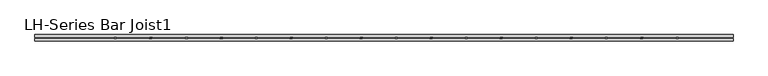
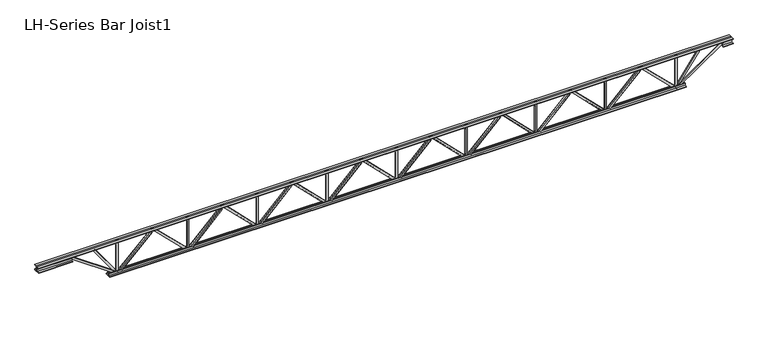
"""IFC4 building model written with IfcOpenShell, lengths in millimetres: beam geometry, LH-Series Bar Joist1 : 32LH-SP1."""

from ifc_helpers import new_model, si_unit, frame, origin, place, context, project, spatial, polyline, outline, extrude, faceted_brep, source, transform, mapped, element, save


def lh_series_bar_joist1_80182e71(model_context):
    return source(origin(), model_context, "Body", "SolidModel", [
        extrude(outline(polyline([(406.4, 3276.6), (406.4, 3225.8), (323.85, 3225.8), (312.7375, 3236.9125), (-312.7375, 3236.9125), (-323.85, 3225.8), (-406.4, 3225.8), (-406.4, 3276.6), (406.4, 3276.6)])), frame((0.0, -12.7, 0.0), z_axis=(0.0, 1.0, 0.0), x_axis=(0.0, 0.0, 1.0)), (0.0, 0.0, 1.0), 25.4),
        faceted_brep([(3251.2, 0.0, -355.6), (3251.2, 0.0, -406.4), (3251.2, 12.7, -406.4), (3251.2, 12.7, -355.6), (3236.3210245, 0.0, -355.6), (2474.3210245, 0.0, 406.4), (2413.0, 0.0, 406.4), (2413.0, 0.0, 355.6), (2453.2789755, 0.0, 355.6), (3215.2789755, 0.0, -406.4), (3215.2789755, 12.7, -406.4), (3151.7789755, 12.7, -342.9), (3160.7592316, 12.7, -333.9197439), (2474.9592316, 12.7, 351.8802561), (2465.9789755, 12.7, 342.9), (2453.2789755, 12.7, 355.6), (2413.0, 12.7, 355.6), (2413.0, 12.7, 406.4), (2474.3210245, 12.7, 406.4), (3236.3210245, 12.7, -355.6), (2465.9789755, 50.8, 342.9), (3151.7789755, 50.8, -342.9), (3160.7592316, 50.8, -333.9197439), (2474.9592316, 50.8, 351.8802561)], [[[0, 1, 2, 3]], [[1, 0, 4, 5, 6, 7, 8, 9]], [[2, 1, 9, 10]], [[3, 2, 10, 11, 12, 13, 14, 15, 16, 17, 18, 19]], [[0, 3, 19, 4]], [[9, 8, 15, 14, 20, 21, 11, 10]], [[5, 4, 19, 18]], [[7, 6, 17, 16]], [[8, 7, 16, 15]], [[6, 5, 18, 17]], [[11, 21, 22, 12]], [[13, 23, 20, 14]], [[22, 21, 20, 23]], [[12, 22, 23, 13]]]),
        faceted_brep([(1625.6, -12.7, -355.6), (1625.6, 0.0, -355.6), (1625.6, 0.0, -406.4), (1625.6, -12.7, -406.4), (1640.4789755, -12.7, -355.6), (1640.4789755, 0.0, -355.6), (2402.4789755, 0.0, 406.4), (2463.8, 0.0, 406.4), (2463.8, 0.0, 355.6), (2423.5210245, 0.0, 355.6), (1661.5210245, 0.0, -406.4), (1661.5210245, -12.7, -406.4), (1725.0210245, -12.7, -342.9), (1716.0407684, -12.7, -333.9197439), (2401.8407684, -12.7, 351.8802561), (2410.8210245, -12.7, 342.9), (2423.5210245, -12.7, 355.6), (2463.8, -12.7, 355.6), (2463.8, -12.7, 406.4), (2402.4789755, -12.7, 406.4), (2410.8210245, -50.8, 342.9), (1725.0210245, -50.8, -342.9), (1716.0407684, -50.8, -333.9197439), (2401.8407684, -50.8, 351.8802561)], [[[0, 1, 2, 3]], [[1, 0, 4, 5]], [[2, 1, 5, 6, 7, 8, 9, 10]], [[3, 2, 10, 11]], [[0, 3, 11, 12, 13, 14, 15, 16, 17, 18, 19, 4]], [[5, 4, 19, 6]], [[10, 9, 16, 15, 20, 21, 12, 11]], [[8, 7, 18, 17]], [[7, 6, 19, 18]], [[9, 8, 17, 16]], [[21, 22, 13, 12]], [[20, 15, 14, 23]], [[22, 21, 20, 23]], [[13, 22, 23, 14]]]),
        extrude(outline(polyline([(406.4, 1651.0), (406.4, 1600.2), (323.85, 1600.2), (312.7375, 1611.3125), (-312.7375, 1611.3125), (-323.85, 1600.2), (-406.4, 1600.2), (-406.4, 1651.0), (406.4, 1651.0)])), frame((0.0, -12.7, 0.0), z_axis=(0.0, 1.0, 0.0), x_axis=(0.0, 0.0, 1.0)), (0.0, 0.0, 1.0), 25.4),
        faceted_brep([(1625.6, 0.0, -355.6), (1625.6, 0.0, -406.4), (1625.6, 12.7, -406.4), (1625.6, 12.7, -355.6), (1610.7210245, 0.0, -355.6), (848.7210245, 0.0, 406.4), (787.4, 0.0, 406.4), (787.4, 0.0, 355.6), (827.6789755, 0.0, 355.6), (1589.6789755, 0.0, -406.4), (1589.6789755, 12.7, -406.4), (1526.1789755, 12.7, -342.9), (1535.1592316, 12.7, -333.9197439), (849.3592316, 12.7, 351.8802561), (840.3789755, 12.7, 342.9), (827.6789755, 12.7, 355.6), (787.4, 12.7, 355.6), (787.4, 12.7, 406.4), (848.7210245, 12.7, 406.4), (1610.7210245, 12.7, -355.6), (840.3789755, 50.8, 342.9), (1526.1789755, 50.8, -342.9), (1535.1592316, 50.8, -333.9197439), (849.3592316, 50.8, 351.8802561)], [[[0, 1, 2, 3]], [[1, 0, 4, 5, 6, 7, 8, 9]], [[2, 1, 9, 10]], [[3, 2, 10, 11, 12, 13, 14, 15, 16, 17, 18, 19]], [[0, 3, 19, 4]], [[9, 8, 15, 14, 20, 21, 11, 10]], [[5, 4, 19, 18]], [[7, 6, 17, 16]], [[8, 7, 16, 15]], [[6, 5, 18, 17]], [[11, 21, 22, 12]], [[13, 23, 20, 14]], [[22, 21, 20, 23]], [[12, 22, 23, 13]]]),
        faceted_brep([(0.0, -12.7, -355.6), (0.0, 0.0, -355.6), (0.0, 0.0, -406.4), (0.0, -12.7, -406.4), (14.8789755, -12.7, -355.6), (14.8789755, 0.0, -355.6), (776.8789755, 0.0, 406.4), (838.2, 0.0, 406.4), (838.2, 0.0, 355.6), (797.9210245, 0.0, 355.6), (35.9210245, 0.0, -406.4), (35.9210245, -12.7, -406.4), (99.4210245, -12.7, -342.9), (90.4407684, -12.7, -333.9197439), (776.2407684, -12.7, 351.8802561), (785.2210245, -12.7, 342.9), (797.9210245, -12.7, 355.6), (838.2, -12.7, 355.6), (838.2, -12.7, 406.4), (776.8789755, -12.7, 406.4), (785.2210245, -50.8, 342.9), (99.4210245, -50.8, -342.9), (90.4407684, -50.8, -333.9197439), (776.2407684, -50.8, 351.8802561)], [[[0, 1, 2, 3]], [[1, 0, 4, 5]], [[2, 1, 5, 6, 7, 8, 9, 10]], [[3, 2, 10, 11]], [[0, 3, 11, 12, 13, 14, 15, 16, 17, 18, 19, 4]], [[5, 4, 19, 6]], [[10, 9, 16, 15, 20, 21, 12, 11]], [[8, 7, 18, 17]], [[7, 6, 19, 18]], [[9, 8, 17, 16]], [[21, 22, 13, 12]], [[20, 15, 14, 23]], [[22, 21, 20, 23]], [[13, 22, 23, 14]]]),
        extrude(outline(polyline([(406.4, 25.4), (406.4, -25.4), (323.85, -25.4), (312.7375, -14.2875), (-312.7375, -14.2875), (-323.85, -25.4), (-406.4, -25.4), (-406.4, 25.4), (406.4, 25.4)])), frame((0.0, -12.7, 0.0), z_axis=(0.0, 1.0, 0.0), x_axis=(0.0, 0.0, 1.0)), (0.0, 0.0, 1.0), 25.4),
        faceted_brep([(0.0, 0.0, -355.6), (0.0, 0.0, -406.4), (0.0, 12.7, -406.4), (0.0, 12.7, -355.6), (-14.8789755, 0.0, -355.6), (-776.8789755, 0.0, 406.4), (-838.2, 0.0, 406.4), (-838.2, 0.0, 355.6), (-797.9210245, 0.0, 355.6), (-35.9210245, 0.0, -406.4), (-35.9210245, 12.7, -406.4), (-99.4210245, 12.7, -342.9), (-90.4407684, 12.7, -333.9197439), (-776.2407684, 12.7, 351.8802561), (-785.2210245, 12.7, 342.9), (-797.9210245, 12.7, 355.6), (-838.2, 12.7, 355.6), (-838.2, 12.7, 406.4), (-776.8789755, 12.7, 406.4), (-14.8789755, 12.7, -355.6), (-785.2210245, 50.8, 342.9), (-99.4210245, 50.8, -342.9), (-90.4407684, 50.8, -333.9197439), (-776.2407684, 50.8, 351.8802561)], [[[0, 1, 2, 3]], [[1, 0, 4, 5, 6, 7, 8, 9]], [[2, 1, 9, 10]], [[3, 2, 10, 11, 12, 13, 14, 15, 16, 17, 18, 19]], [[0, 3, 19, 4]], [[9, 8, 15, 14, 20, 21, 11, 10]], [[5, 4, 19, 18]], [[7, 6, 17, 16]], [[8, 7, 16, 15]], [[6, 5, 18, 17]], [[11, 21, 22, 12]], [[13, 23, 20, 14]], [[22, 21, 20, 23]], [[12, 22, 23, 13]]]),
        faceted_brep([(-1625.6, -12.7, -355.6), (-1625.6, 0.0, -355.6), (-1625.6, 0.0, -406.4), (-1625.6, -12.7, -406.4), (-1610.7210245, -12.7, -355.6), (-1610.7210245, 0.0, -355.6), (-848.7210245, 0.0, 406.4), (-787.4, 0.0, 406.4), (-787.4, 0.0, 355.6), (-827.6789755, 0.0, 355.6), (-1589.6789755, 0.0, -406.4), (-1589.6789755, -12.7, -406.4), (-1526.1789755, -12.7, -342.9), (-1535.1592316, -12.7, -333.9197439), (-849.3592316, -12.7, 351.8802561), (-840.3789755, -12.7, 342.9), (-827.6789755, -12.7, 355.6), (-787.4, -12.7, 355.6), (-787.4, -12.7, 406.4), (-848.7210245, -12.7, 406.4), (-840.3789755, -50.8, 342.9), (-1526.1789755, -50.8, -342.9), (-1535.1592316, -50.8, -333.9197439), (-849.3592316, -50.8, 351.8802561)], [[[0, 1, 2, 3]], [[1, 0, 4, 5]], [[2, 1, 5, 6, 7, 8, 9, 10]], [[3, 2, 10, 11]], [[0, 3, 11, 12, 13, 14, 15, 16, 17, 18, 19, 4]], [[5, 4, 19, 6]], [[10, 9, 16, 15, 20, 21, 12, 11]], [[8, 7, 18, 17]], [[7, 6, 19, 18]], [[9, 8, 17, 16]], [[21, 22, 13, 12]], [[20, 15, 14, 23]], [[22, 21, 20, 23]], [[13, 22, 23, 14]]]),
        extrude(outline(polyline([(406.4, 6556.375), (406.4, 6505.575), (323.85, 6505.575), (312.7375, 6516.6875), (-312.7375, 6516.6875), (-323.85, 6505.575), (-406.4, 6505.575), (-406.4, 6556.375), (406.4, 6556.375)])), frame((0.0, -12.7, 0.0), z_axis=(0.0, 1.0, 0.0), x_axis=(0.0, 0.0, 1.0)), (0.0, 0.0, 1.0), 25.4),
        faceted_brep([(6530.975, 0.0, -355.6), (6530.975, 0.0, -406.4), (6530.975, 12.7, -406.4), (6530.975, 12.7, -355.6), (6515.958098, 0.0, -355.6), (5739.670598, 0.0, 406.4), (5678.4875, 0.0, 406.4), (5678.4875, 0.0, 355.6), (5718.904402, 0.0, 355.6), (6495.191902, 0.0, -406.4), (6495.191902, 12.7, -406.4), (6431.104883, 12.7, -343.4924966), (6440.0013474, 12.7, -334.4292234), (5740.6182703, 12.7, 352.0817725), (5731.7218059, 12.7, 343.0184993), (5718.904402, 12.7, 355.6), (5678.4875, 12.7, 355.6), (5678.4875, 12.7, 406.4), (5739.670598, 12.7, 406.4), (6515.958098, 12.7, -355.6), (5731.7218059, 50.8, 343.0184993), (6431.104883, 50.8, -343.4924966), (6440.0013474, 50.8, -334.4292234), (5740.6182703, 50.8, 352.0817725)], [[[0, 1, 2, 3]], [[1, 0, 4, 5, 6, 7, 8, 9]], [[2, 1, 9, 10]], [[3, 2, 10, 11, 12, 13, 14, 15, 16, 17, 18, 19]], [[0, 3, 19, 4]], [[9, 8, 15, 14, 20, 21, 11, 10]], [[5, 4, 19, 18]], [[7, 6, 17, 16]], [[8, 7, 16, 15]], [[6, 5, 18, 17]], [[11, 21, 22, 12]], [[13, 23, 20, 14]], [[22, 21, 20, 23]], [[12, 22, 23, 13]]]),
        faceted_brep([(4876.8, -12.7, -355.6), (4876.8, 0.0, -355.6), (4876.8, 0.0, -406.4), (4876.8, -12.7, -406.4), (4891.816902, -12.7, -355.6), (4891.816902, 0.0, -355.6), (5668.104402, 0.0, 406.4), (5729.2875, 0.0, 406.4), (5729.2875, 0.0, 355.6), (5688.870598, 0.0, 355.6), (4912.583098, 0.0, -406.4), (4912.583098, -12.7, -406.4), (4976.670117, -12.7, -343.4924966), (4967.7736526, -12.7, -334.4292234), (5667.1567297, -12.7, 352.0817725), (5676.0531941, -12.7, 343.0184993), (5688.870598, -12.7, 355.6), (5729.2875, -12.7, 355.6), (5729.2875, -12.7, 406.4), (5668.104402, -12.7, 406.4), (5676.0531941, -50.8, 343.0184993), (4976.670117, -50.8, -343.4924966), (4967.7736526, -50.8, -334.4292234), (5667.1567297, -50.8, 352.0817725)], [[[0, 1, 2, 3]], [[1, 0, 4, 5]], [[2, 1, 5, 6, 7, 8, 9, 10]], [[3, 2, 10, 11]], [[0, 3, 11, 12, 13, 14, 15, 16, 17, 18, 19, 4]], [[5, 4, 19, 6]], [[10, 9, 16, 15, 20, 21, 12, 11]], [[8, 7, 18, 17]], [[7, 6, 19, 18]], [[9, 8, 17, 16]], [[21, 22, 13, 12]], [[20, 15, 14, 23]], [[22, 21, 20, 23]], [[13, 22, 23, 14]]]),
        extrude(outline(polyline([(406.4, -4851.4), (406.4, -4902.2), (323.85, -4902.2), (312.7375, -4891.0875), (-312.7375, -4891.0875), (-323.85, -4902.2), (-406.4, -4902.2), (-406.4, -4851.4), (406.4, -4851.4)])), frame((0.0, -12.7, 0.0), z_axis=(0.0, 1.0, 0.0), x_axis=(0.0, 0.0, 1.0)), (0.0, 0.0, 1.0), 25.4),
        extrude(outline(polyline([(406.4, -6505.575), (406.4, -6556.375), (323.85, -6556.375), (312.7375, -6545.2625), (-312.7375, -6545.2625), (-323.85, -6556.375), (-406.4, -6556.375), (-406.4, -6505.575), (406.4, -6505.575)])), frame((0.0, -12.7, 0.0), z_axis=(0.0, 1.0, 0.0), x_axis=(0.0, 0.0, 1.0)), (0.0, 0.0, 1.0), 25.4),
        faceted_brep([(-4876.8, 0.0, -355.6), (-4876.8, 0.0, -406.4), (-4876.8, 12.7, -406.4), (-4876.8, 12.7, -355.6), (-4891.816902, 0.0, -355.6), (-5668.104402, 0.0, 406.4), (-5729.2875, 0.0, 406.4), (-5729.2875, 0.0, 355.6), (-5688.870598, 0.0, 355.6), (-4912.583098, 0.0, -406.4), (-4912.583098, 12.7, -406.4), (-4976.670117, 12.7, -343.4924966), (-4967.7736526, 12.7, -334.4292234), (-5667.1567297, 12.7, 352.0817725), (-5676.0531941, 12.7, 343.0184993), (-5688.870598, 12.7, 355.6), (-5729.2875, 12.7, 355.6), (-5729.2875, 12.7, 406.4), (-5668.104402, 12.7, 406.4), (-4891.816902, 12.7, -355.6), (-5676.0531941, 50.8, 343.0184993), (-4976.670117, 50.8, -343.4924966), (-4967.7736526, 50.8, -334.4292234), (-5667.1567297, 50.8, 352.0817725)], [[[0, 1, 2, 3]], [[1, 0, 4, 5, 6, 7, 8, 9]], [[2, 1, 9, 10]], [[3, 2, 10, 11, 12, 13, 14, 15, 16, 17, 18, 19]], [[0, 3, 19, 4]], [[9, 8, 15, 14, 20, 21, 11, 10]], [[5, 4, 19, 18]], [[7, 6, 17, 16]], [[8, 7, 16, 15]], [[6, 5, 18, 17]], [[11, 21, 22, 12]], [[13, 23, 20, 14]], [[22, 21, 20, 23]], [[12, 22, 23, 13]]]),
        faceted_brep([(-6530.975, -12.7, -355.6), (-6530.975, 0.0, -355.6), (-6530.975, 0.0, -406.4), (-6530.975, -12.7, -406.4), (-6515.958098, -12.7, -355.6), (-6515.958098, 0.0, -355.6), (-5739.670598, 0.0, 406.4), (-5678.4875, 0.0, 406.4), (-5678.4875, 0.0, 355.6), (-5718.904402, 0.0, 355.6), (-6495.191902, 0.0, -406.4), (-6495.191902, -12.7, -406.4), (-6431.104883, -12.7, -343.4924966), (-6440.0013474, -12.7, -334.4292234), (-5740.6182703, -12.7, 352.0817725), (-5731.7218059, -12.7, 343.0184993), (-5718.904402, -12.7, 355.6), (-5678.4875, -12.7, 355.6), (-5678.4875, -12.7, 406.4), (-5739.670598, -12.7, 406.4), (-5731.7218059, -50.8, 343.0184993), (-6431.104883, -50.8, -343.4924966), (-6440.0013474, -50.8, -334.4292234), (-5740.6182703, -50.8, 352.0817725)], [[[0, 1, 2, 3]], [[1, 0, 4, 5]], [[2, 1, 5, 6, 7, 8, 9, 10]], [[3, 2, 10, 11]], [[0, 3, 11, 12, 13, 14, 15, 16, 17, 18, 19, 4]], [[5, 4, 19, 6]], [[10, 9, 16, 15, 20, 21, 12, 11]], [[8, 7, 18, 17]], [[7, 6, 19, 18]], [[9, 8, 17, 16]], [[21, 22, 13, 12]], [[20, 15, 14, 23]], [[22, 21, 20, 23]], [[13, 22, 23, 14]]]),
        extrude(outline(polyline([(406.4, -1600.2), (406.4, -1651.0), (323.85, -1651.0), (312.7375, -1639.8875), (-312.7375, -1639.8875), (-323.85, -1651.0), (-406.4, -1651.0), (-406.4, -1600.2), (406.4, -1600.2)])), frame((0.0, -12.7, 0.0), z_axis=(0.0, 1.0, 0.0), x_axis=(0.0, 0.0, 1.0)), (0.0, 0.0, 1.0), 25.4),
        faceted_brep([(-1625.6, 0.0, -355.6), (-1625.6, 0.0, -406.4), (-1625.6, 12.7, -406.4), (-1625.6, 12.7, -355.6), (-1640.4789755, 0.0, -355.6), (-2402.4789755, 0.0, 406.4), (-2463.8, 0.0, 406.4), (-2463.8, 0.0, 355.6), (-2423.5210245, 0.0, 355.6), (-1661.5210245, 0.0, -406.4), (-1661.5210245, 12.7, -406.4), (-1725.0210245, 12.7, -342.9), (-1716.0407684, 12.7, -333.9197439), (-2401.8407684, 12.7, 351.8802561), (-2410.8210245, 12.7, 342.9), (-2423.5210245, 12.7, 355.6), (-2463.8, 12.7, 355.6), (-2463.8, 12.7, 406.4), (-2402.4789755, 12.7, 406.4), (-1640.4789755, 12.7, -355.6), (-2410.8210245, 50.8, 342.9), (-1725.0210245, 50.8, -342.9), (-1716.0407684, 50.8, -333.9197439), (-2401.8407684, 50.8, 351.8802561)], [[[0, 1, 2, 3]], [[1, 0, 4, 5, 6, 7, 8, 9]], [[2, 1, 9, 10]], [[3, 2, 10, 11, 12, 13, 14, 15, 16, 17, 18, 19]], [[0, 3, 19, 4]], [[9, 8, 15, 14, 20, 21, 11, 10]], [[5, 4, 19, 18]], [[7, 6, 17, 16]], [[8, 7, 16, 15]], [[6, 5, 18, 17]], [[11, 21, 22, 12]], [[13, 23, 20, 14]], [[22, 21, 20, 23]], [[12, 22, 23, 13]]]),
        faceted_brep([(-3251.2, -12.7, -355.6), (-3251.2, 0.0, -355.6), (-3251.2, 0.0, -406.4), (-3251.2, -12.7, -406.4), (-3236.3210245, -12.7, -355.6), (-3236.3210245, 0.0, -355.6), (-2474.3210245, 0.0, 406.4), (-2413.0, 0.0, 406.4), (-2413.0, 0.0, 355.6), (-2453.2789755, 0.0, 355.6), (-3215.2789755, 0.0, -406.4), (-3215.2789755, -12.7, -406.4), (-3151.7789755, -12.7, -342.9), (-3160.7592316, -12.7, -333.9197439), (-2474.9592316, -12.7, 351.8802561), (-2465.9789755, -12.7, 342.9), (-2453.2789755, -12.7, 355.6), (-2413.0, -12.7, 355.6), (-2413.0, -12.7, 406.4), (-2474.3210245, -12.7, 406.4), (-2465.9789755, -50.8, 342.9), (-3151.7789755, -50.8, -342.9), (-3160.7592316, -50.8, -333.9197439), (-2474.9592316, -50.8, 351.8802561)], [[[0, 1, 2, 3]], [[1, 0, 4, 5]], [[2, 1, 5, 6, 7, 8, 9, 10]], [[3, 2, 10, 11]], [[0, 3, 11, 12, 13, 14, 15, 16, 17, 18, 19, 4]], [[5, 4, 19, 6]], [[10, 9, 16, 15, 20, 21, 12, 11]], [[8, 7, 18, 17]], [[7, 6, 19, 18]], [[9, 8, 17, 16]], [[21, 22, 13, 12]], [[20, 15, 14, 23]], [[22, 21, 20, 23]], [[13, 22, 23, 14]]]),
        extrude(outline(polyline([(406.4, 4902.2), (406.4, 4851.4), (323.85, 4851.4), (312.7375, 4862.5125), (-312.7375, 4862.5125), (-323.85, 4851.4), (-406.4, 4851.4), (-406.4, 4902.2), (406.4, 4902.2)])), frame((0.0, -12.7, 0.0), z_axis=(0.0, 1.0, 0.0), x_axis=(0.0, 0.0, 1.0)), (0.0, 0.0, 1.0), 25.4),
        faceted_brep([(4876.8, 0.0, -355.6), (4876.8, 0.0, -406.4), (4876.8, 12.7, -406.4), (4876.8, 12.7, -355.6), (4861.9210245, 0.0, -355.6), (4099.9210245, 0.0, 406.4), (4038.6, 0.0, 406.4), (4038.6, 0.0, 355.6), (4078.8789755, 0.0, 355.6), (4840.8789755, 0.0, -406.4), (4840.8789755, 12.7, -406.4), (4777.3789755, 12.7, -342.9), (4786.3592316, 12.7, -333.9197439), (4100.5592316, 12.7, 351.8802561), (4091.5789755, 12.7, 342.9), (4078.8789755, 12.7, 355.6), (4038.6, 12.7, 355.6), (4038.6, 12.7, 406.4), (4099.9210245, 12.7, 406.4), (4861.9210245, 12.7, -355.6), (4091.5789755, 50.8, 342.9), (4777.3789755, 50.8, -342.9), (4786.3592316, 50.8, -333.9197439), (4100.5592316, 50.8, 351.8802561)], [[[0, 1, 2, 3]], [[1, 0, 4, 5, 6, 7, 8, 9]], [[2, 1, 9, 10]], [[3, 2, 10, 11, 12, 13, 14, 15, 16, 17, 18, 19]], [[0, 3, 19, 4]], [[9, 8, 15, 14, 20, 21, 11, 10]], [[5, 4, 19, 18]], [[7, 6, 17, 16]], [[8, 7, 16, 15]], [[6, 5, 18, 17]], [[11, 21, 22, 12]], [[13, 23, 20, 14]], [[22, 21, 20, 23]], [[12, 22, 23, 13]]]),
        faceted_brep([(3251.2, -12.7, -355.6), (3251.2, 0.0, -355.6), (3251.2, 0.0, -406.4), (3251.2, -12.7, -406.4), (3266.0789755, -12.7, -355.6), (3266.0789755, 0.0, -355.6), (4028.0789755, 0.0, 406.4), (4089.4, 0.0, 406.4), (4089.4, 0.0, 355.6), (4049.1210245, 0.0, 355.6), (3287.1210245, 0.0, -406.4), (3287.1210245, -12.7, -406.4), (3350.6210245, -12.7, -342.9), (3341.6407684, -12.7, -333.9197439), (4027.4407684, -12.7, 351.8802561), (4036.4210245, -12.7, 342.9), (4049.1210245, -12.7, 355.6), (4089.4, -12.7, 355.6), (4089.4, -12.7, 406.4), (4028.0789755, -12.7, 406.4), (4036.4210245, -50.8, 342.9), (3350.6210245, -50.8, -342.9), (3341.6407684, -50.8, -333.9197439), (4027.4407684, -50.8, 351.8802561)], [[[0, 1, 2, 3]], [[1, 0, 4, 5]], [[2, 1, 5, 6, 7, 8, 9, 10]], [[3, 2, 10, 11]], [[0, 3, 11, 12, 13, 14, 15, 16, 17, 18, 19, 4]], [[5, 4, 19, 6]], [[10, 9, 16, 15, 20, 21, 12, 11]], [[8, 7, 18, 17]], [[7, 6, 19, 18]], [[9, 8, 17, 16]], [[21, 22, 13, 12]], [[20, 15, 14, 23]], [[22, 21, 20, 23]], [[13, 22, 23, 14]]]),
        extrude(outline(polyline([(406.4, -3225.8), (406.4, -3276.6), (323.85, -3276.6), (312.7375, -3265.4875), (-312.7375, -3265.4875), (-323.85, -3276.6), (-406.4, -3276.6), (-406.4, -3225.8), (406.4, -3225.8)])), frame((0.0, -12.7, 0.0), z_axis=(0.0, 1.0, 0.0), x_axis=(0.0, 0.0, 1.0)), (0.0, 0.0, 1.0), 25.4),
        faceted_brep([(-3251.2, 0.0, -355.6), (-3251.2, 0.0, -406.4), (-3251.2, 12.7, -406.4), (-3251.2, 12.7, -355.6), (-3266.0789755, 0.0, -355.6), (-4028.0789755, 0.0, 406.4), (-4089.4, 0.0, 406.4), (-4089.4, 0.0, 355.6), (-4049.1210245, 0.0, 355.6), (-3287.1210245, 0.0, -406.4), (-3287.1210245, 12.7, -406.4), (-3350.6210245, 12.7, -342.9), (-3341.6407684, 12.7, -333.9197439), (-4027.4407684, 12.7, 351.8802561), (-4036.4210245, 12.7, 342.9), (-4049.1210245, 12.7, 355.6), (-4089.4, 12.7, 355.6), (-4089.4, 12.7, 406.4), (-4028.0789755, 12.7, 406.4), (-3266.0789755, 12.7, -355.6), (-4036.4210245, 50.8, 342.9), (-3350.6210245, 50.8, -342.9), (-3341.6407684, 50.8, -333.9197439), (-4027.4407684, 50.8, 351.8802561)], [[[0, 1, 2, 3]], [[1, 0, 4, 5, 6, 7, 8, 9]], [[2, 1, 9, 10]], [[3, 2, 10, 11, 12, 13, 14, 15, 16, 17, 18, 19]], [[0, 3, 19, 4]], [[9, 8, 15, 14, 20, 21, 11, 10]], [[5, 4, 19, 18]], [[7, 6, 17, 16]], [[8, 7, 16, 15]], [[6, 5, 18, 17]], [[11, 21, 22, 12]], [[13, 23, 20, 14]], [[22, 21, 20, 23]], [[12, 22, 23, 13]]]),
        faceted_brep([(-4876.8, -12.7, -355.6), (-4876.8, 0.0, -355.6), (-4876.8, 0.0, -406.4), (-4876.8, -12.7, -406.4), (-4861.9210245, -12.7, -355.6), (-4861.9210245, 0.0, -355.6), (-4099.9210245, 0.0, 406.4), (-4038.6, 0.0, 406.4), (-4038.6, 0.0, 355.6), (-4078.8789755, 0.0, 355.6), (-4840.8789755, 0.0, -406.4), (-4840.8789755, -12.7, -406.4), (-4777.3789755, -12.7, -342.9), (-4786.3592316, -12.7, -333.9197439), (-4100.5592316, -12.7, 351.8802561), (-4091.5789755, -12.7, 342.9), (-4078.8789755, -12.7, 355.6), (-4038.6, -12.7, 355.6), (-4038.6, -12.7, 406.4), (-4099.9210245, -12.7, 406.4), (-4091.5789755, -50.8, 342.9), (-4777.3789755, -50.8, -342.9), (-4786.3592316, -50.8, -333.9197439), (-4100.5592316, -50.8, 351.8802561)], [[[0, 1, 2, 3]], [[1, 0, 4, 5]], [[2, 1, 5, 6, 7, 8, 9, 10]], [[3, 2, 10, 11]], [[0, 3, 11, 12, 13, 14, 15, 16, 17, 18, 19, 4]], [[5, 4, 19, 6]], [[10, 9, 16, 15, 20, 21, 12, 11]], [[8, 7, 18, 17]], [[7, 6, 19, 18]], [[9, 8, 17, 16]], [[21, 22, 13, 12]], [[20, 15, 14, 23]], [[22, 21, 20, 23]], [[13, 22, 23, 14]]]),
        extrude(outline(polyline([(12.7, 406.4), (76.2, 406.4), (76.2, 393.7), (25.4, 393.7), (25.4, 342.9), (12.7, 342.9), (12.7, 406.4)])), frame((-8397.875, 0.0, 0.0), z_axis=(1.0, 0.0, 0.0), x_axis=(0.0, 1.0, 0.0)), (0.0, 0.0, 1.0), 16224.25),
        extrude(outline(polyline([(-12.7, 406.4), (-12.7, 342.9), (-25.4, 342.9), (-25.4, 393.7), (-76.2, 393.7), (-76.2, 406.4), (-12.7, 406.4)])), frame((-8397.875, 0.0, 0.0), z_axis=(1.0, 0.0, 0.0), x_axis=(0.0, 1.0, 0.0)), (0.0, 0.0, 1.0), 16224.25),
        extrude(outline(polyline([(-12.7, 279.4), (-76.2, 279.4), (-76.2, 292.1), (-25.4, 292.1), (-25.4, 342.9), (-12.7, 342.9), (-12.7, 279.4)])), frame((-8397.875, 0.0, 0.0), z_axis=(1.0, 0.0, 0.0), x_axis=(0.0, 1.0, 0.0)), (0.0, 0.0, 1.0), 800.1),
        extrude(outline(polyline([(76.2, 279.4), (12.7, 279.4), (12.7, 342.9), (25.4, 342.9), (25.4, 292.1), (76.2, 292.1), (76.2, 279.4)])), frame((-8397.875, 0.0, 0.0), z_axis=(1.0, 0.0, 0.0), x_axis=(0.0, 1.0, 0.0)), (0.0, 0.0, 1.0), 800.1),
        extrude(outline(polyline([(12.7, 279.4), (12.7, 342.9), (25.4, 342.9), (25.4, 292.1), (76.2, 292.1), (76.2, 279.4), (12.7, 279.4)])), frame((7597.775, 0.0, 0.0), z_axis=(1.0, 0.0, 0.0), x_axis=(0.0, 1.0, 0.0)), (0.0, 0.0, 1.0), 228.6),
        extrude(outline(polyline([(-12.7, 279.4), (-76.2, 279.4), (-76.2, 292.1), (-25.4, 292.1), (-25.4, 342.9), (-12.7, 342.9), (-12.7, 279.4)])), frame((7597.775, 0.0, 0.0), z_axis=(1.0, 0.0, 0.0), x_axis=(0.0, 1.0, 0.0)), (0.0, 0.0, 1.0), 228.6),
        extrude(outline(polyline([(12.7, -406.4), (12.7, -342.9), (25.4, -342.9), (25.4, -393.7), (76.2, -393.7), (76.2, -406.4), (12.7, -406.4)])), frame((-6734.175, 0.0, 0.0), z_axis=(1.0, 0.0, 0.0), x_axis=(0.0, 1.0, 0.0)), (0.0, 0.0, 1.0), 13468.35),
        extrude(outline(polyline([(-12.7, -406.4), (-76.2, -406.4), (-76.2, -393.7), (-25.4, -393.7), (-25.4, -342.9), (-12.7, -342.9), (-12.7, -406.4)])), frame((-6734.175, 0.0, 0.0), z_axis=(1.0, 0.0, 0.0), x_axis=(0.0, 1.0, 0.0)), (0.0, 0.0, 1.0), 13468.35),
        extrude(outline(polyline([(6.35, -25.4), (-6.35, -25.4), (-6.35, 25.4), (6.35, 25.4), (6.35, -25.4)])), frame((-6530.975, 0.0, -400.05), z_axis=(-0.58320678309139, 0.0, 0.8123237335915974), x_axis=(0.0, -1.0, 0.0)), (0.0, 0.0, 1.0), 914.598416),
        extrude(outline(polyline([(0.0, -12.7), (0.0, 0.0), (1300.0142086, 0.0), (1300.0142086, -12.7), (0.0, -12.7)])), frame((-7612.2909413, 6.35, 322.056597), z_axis=(0.5714937537595753, 0.0, 0.8206064156547828), x_axis=(0.8206064156547828, 0.0, -0.5714937537595753)), (0.0, 0.0, 1.0), 50.8),
        extrude(outline(polyline([(6.35, 25.4), (6.35, -25.4), (-6.35, -25.4), (-6.35, 25.4), (6.35, 25.4)])), frame((6530.975, 0.0, -400.05), z_axis=(0.5811065900870399, 0.0, 0.8138274577313137), x_axis=(0.0, -1.0, 0.0)), (0.0, 0.0, 1.0), 912.9084955),
        extrude(outline(polyline([(0.0, -12.7), (0.0, 0.0), (1300.0142086, 0.0), (1300.0142086, -12.7), (0.0, -12.7)])), frame((6545.4909413, -6.35, -420.893403), z_axis=(-0.5714937537593278, 0.0, 0.8206064156549552), x_axis=(0.8206064156549552, 0.0, 0.5714937537593278)), (0.0, 0.0, 1.0), 50.8),
    ])


if __name__ == "__main__":
    model = new_model("IFC4")
    model_context = context("Model", 3, world=origin())
    ifc_project = project(units=[si_unit("LENGTHUNIT", "METRE", prefix="MILLI")], contexts=[model_context])
    site = spatial("IfcSite", under=ifc_project)
    building = spatial("IfcBuilding", under=site)
    placement = place(None, origin())
    lh_series_bar_joist1_shape = lh_series_bar_joist1_80182e71(model_context)
    element("IfcBeam", 1, ObjectType="LH-Series Bar Joist1 : 32LH-SP1", at=placement, inside=building, context=model_context, shape_type="MappedRepresentation", body=[
        mapped(lh_series_bar_joist1_shape, transform((0.0, 0.0, 0.0), x_axis=(1.0, 0.0, 0.0), y_axis=(0.0, 1.0, 0.0), z_axis=(0.0, 0.0, 1.0))),
    ])
    save(model, "model.ifc")

# Revit data of these elements
# Type "LH-Series Bar Joist1 : 32LH-SP1"
#   Assembly Code = "B1010350"
#   Wt = 21
#   Web Thickness = 0' - 1"
#   Variable Panel [instance default] = 5' - 4"
#   Start Offset [instance default] = 0' - 0"
#   Start Extension [instance default] = 0' - 0"
#   Seat Length = 0' - 6"
#   Seat Depth = 0' - 5"
#   IntPanelWidth [instance default] = 5' - 4"
#   IntPanelArrayLength [instance default] = 21' - 4"
#   PanelAreaLength [instance default] = 32' - 0"
#   End Panel = 4' - 0"
#   End Offset [instance default] = 0' - 0"
#   End Extension [instance default] = 0' - 0"
#   Cord Leg = 0' - 2 1/2"
#   Chord Thickness = 0' - 0 1/2"
#   Length [instance default] = 40' - 0"
#   Depth = 2' - 8"
#   Vertical Member Visibility = yes
#   IntPanelArrayNum [instance default] = 4
#   Structural Material = none
# Element 1 (IfcBeam, "LH-Series Bar Joist1 : 32LH-SP1")
#   Variable Panel = 5' - 5 1/8"
#   Start Extension = 2' - 1 1/2"
#   IntPanelArrayLength = 32' - 0"
#   PanelAreaLength = 42' - 10 1/4"
#   End Extension = 0' - 3"
#   Length = 50' - 10 1/4"
#   IntPanelArrayNum = 6
